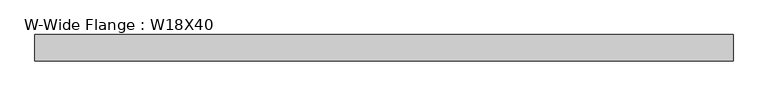
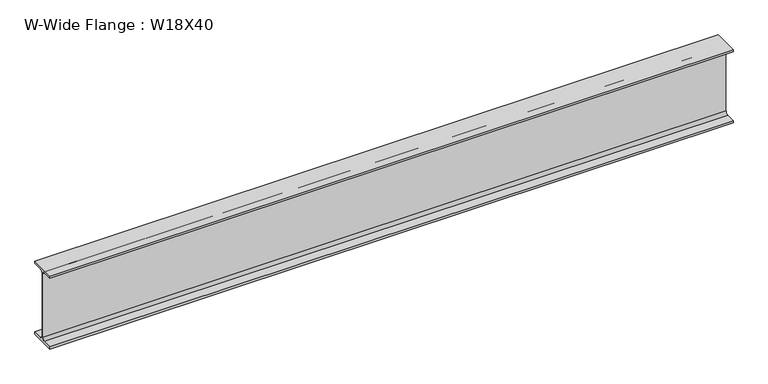
"""IFC4 building model written with IfcOpenShell, lengths in millimetres: beam geometry, W-Wide Flange : W18X40."""

from ifc_helpers import new_model, si_unit, point, frame, frame_2d, origin, place, context, project, spatial, polyline, circle_curve, trimmed, segment, composite_curve, outline, extrude, source, transform, mapped, element, save


def w_wide_flange_w18x40_85a06bf1(model_context):
    return source(origin(), model_context, "Body", "SweptSolid", [
        extrude(outline(composite_curve([segment(polyline([(76.454, -213.995), (76.454, -227.33), (-76.454, -227.33), (-76.454, -213.995), (-20.828, -213.995)]), True, "CONTINUOUS"), segment(trimmed(circle_curve(frame_2d((-20.828, -197.1675)), 16.8275), [point((-20.828, -213.995))], [point((-4.0005, -197.1675))], True, "CARTESIAN"), True, "CONTINUOUS"), segment(polyline([(-4.0005, -197.1675), (-4.0005, 197.1675)]), True, "CONTINUOUS"), segment(trimmed(circle_curve(frame_2d((-20.828, 197.1675)), 16.8275), [point((-4.0005, 197.1675))], [point((-20.828, 213.995))], True, "CARTESIAN"), True, "CONTINUOUS"), segment(polyline([(-20.828, 213.995), (-76.454, 213.995), (-76.454, 227.33), (76.454, 227.33), (76.454, 213.995), (20.828, 213.995)]), True, "CONTINUOUS"), segment(trimmed(circle_curve(frame_2d((20.828, 197.1675)), 16.8275), [point((20.828, 213.995))], [point((4.0005, 197.1675))], True, "CARTESIAN"), True, "CONTINUOUS"), segment(polyline([(4.0005, 197.1675), (4.0005, -197.1675)]), True, "CONTINUOUS"), segment(trimmed(circle_curve(frame_2d((20.828, -197.1675)), 16.8275), [point((4.0005, -197.1675))], [point((20.828, -213.995))], True, "CARTESIAN"), True, "CONTINUOUS"), segment(polyline([(20.828, -213.995), (76.454, -213.995)]), True, "CONTINUOUS")], self_intersect=False)), frame((-2012.95, 0.0, 0.0), z_axis=(1.0, 0.0, 0.0), x_axis=(0.0, 1.0, 0.0)), (0.0, 0.0, 1.0), 4025.9),
    ])


if __name__ == "__main__":
    model = new_model("IFC4")
    model_context = context("Model", 3, world=origin())
    ifc_project = project(units=[si_unit("LENGTHUNIT", "METRE", prefix="MILLI")], contexts=[model_context])
    site = spatial("IfcSite", under=ifc_project)
    building = spatial("IfcBuilding", under=site)
    placement = place(None, origin())
    w_wide_flange_w18x40_shape = w_wide_flange_w18x40_85a06bf1(model_context)
    element("IfcBeam", 1, ObjectType="W-Wide Flange : W18X40", at=placement, inside=building, context=model_context, shape_type="MappedRepresentation", body=[
        mapped(w_wide_flange_w18x40_shape, transform((0.0, 0.0, 0.0), x_axis=(1.0, 0.0, 0.0), y_axis=(0.0, 1.0, 0.0), z_axis=(0.0, 0.0, 1.0))),
    ])
    save(model, "model.ifc")

# Revit data of these elements
# Type "W-Wide Flange : W18X40"
#   Assembly Code = "B10"
#   W = 40
#   Length [instance default] = 5' - 0"
#   bf = 0' - 6.02"
#   d = 1' - 5.9"
#   k = 0' - 1 3/16"
#   k2 = 0' - 0.6625"
#   tf = 0' - 0.525"
#   tw = 0' - 0.315"
#   A = 0.0819444 SF
#   Structural Material [instance default] = Steel ASTM A992
# Element 1 (IfcBeam, "W-Wide Flange : W18X40")
#   Materials on its faces: "Steel ASTM A992"
# Materials
#   "Steel ASTM A992": class "Metal", colour RGB 199 199 199, transparency 0, Description = "Structural steel 50ksi", Cost = 0
